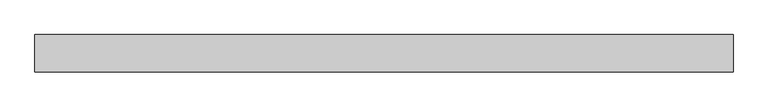
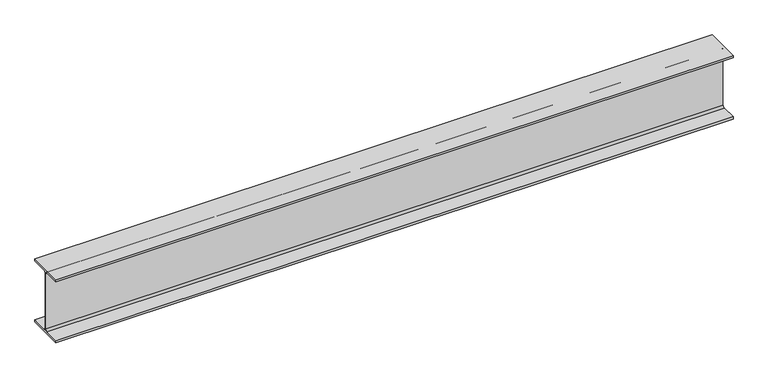
"""IFC4 building model written with IfcOpenShell, lengths in millimetres: beam geometry, Old_Steel Beam_H-KSD3502 : H_SB_ASB_H-300×300x10x15."""

from ifc_helpers import new_model, si_unit, point, frame, frame_2d, origin, place, context, project, spatial, polyline, circle_curve, trimmed, segment, composite_curve, outline, extrude, source, transform, mapped, element, save


def beam_b6f05fa2(model_context):
    return source(origin(), model_context, "Body", "SweptSolid", [
        extrude(outline(composite_curve([segment(polyline([(82.5, -141.5), (82.5, -151.7), (-82.5, -151.7), (-82.5, -141.5), (-11.9, -141.5)]), True, "CONTINUOUS"), segment(trimmed(circle_curve(frame_2d((-11.9, -132.6)), 8.9), [point((-11.9, -141.5))], [point((-3.0, -132.6))], True, "CARTESIAN"), True, "CONTINUOUS"), segment(polyline([(-3.0, -132.6), (-3.0, 132.6)]), True, "CONTINUOUS"), segment(trimmed(circle_curve(frame_2d((-11.9, 132.6)), 8.9), [point((-3.0, 132.6))], [point((-11.9, 141.5))], True, "CARTESIAN"), True, "CONTINUOUS"), segment(polyline([(-11.9, 141.5), (-82.5, 141.5), (-82.5, 151.7), (82.5, 151.7), (82.5, 141.5), (11.9, 141.5)]), True, "CONTINUOUS"), segment(trimmed(circle_curve(frame_2d((11.9, 132.6)), 8.9), [point((11.9, 141.5))], [point((3.0, 132.6))], True, "CARTESIAN"), True, "CONTINUOUS"), segment(polyline([(3.0, 132.6), (3.0, -132.6)]), True, "CONTINUOUS"), segment(trimmed(circle_curve(frame_2d((11.9, -132.6)), 8.9), [point((3.0, -132.6))], [point((11.9, -141.5))], True, "CARTESIAN"), True, "CONTINUOUS"), segment(polyline([(11.9, -141.5), (82.5, -141.5)]), True, "CONTINUOUS")], self_intersect=False)), frame((-1364.2332089, 0.0, 0.0), z_axis=(1.0, 0.0, 0.0), x_axis=(0.0, 1.0, 0.0)), (0.0, 0.0, 1.0), 3068.3751225),
    ])


if __name__ == "__main__":
    model = new_model("IFC4")
    model_context = context("Model", 3, world=origin())
    ifc_project = project(units=[si_unit("LENGTHUNIT", "METRE", prefix="MILLI")], contexts=[model_context])
    site = spatial("IfcSite", under=ifc_project)
    building = spatial("IfcBuilding", under=site)
    placement = place(None, origin())
    beam_shape = beam_b6f05fa2(model_context)
    element("IfcBeam", 1, ObjectType="Old_Steel Beam_H-KSD3502 : H_SB_ASB_H-300×300x10x15", at=placement, inside=building, context=model_context, shape_type="MappedRepresentation", body=[
        mapped(beam_shape, transform((0.0, 0.0, 0.0), x_axis=(1.0, 0.0, 0.0), y_axis=(0.0, 1.0, 0.0), z_axis=(0.0, 0.0, 1.0))),
    ])
    save(model, "model.ifc")

# Revit data of these elements
# Type "Old_Steel Beam_H-KSD3502 : H_SB_ASB_H-300×300x10x15"
#   Width = 30.0 cm
#   Web Thickness = 1.0 cm
#   Web Fillet = 1.8 cm
#   Warping Constant = 1370670.0 cm⁶
#   Torsional Moment of Inertia = 77.00 cm⁴
#   Torsional Modulus = 1.0 cm³
#   Section Area = 119.8 cm²
#   Plastic Modulus weak axis = 684.0 cm³
#   Plastic Modulus strong axis = 1500.0 cm³
#   Perimeter = 1.75 m²/m
#   Nominal Weight = 94.00 kgf/m
#   Moment of Inertia weak axis = 6750.00 cm⁴
#   Moment of Inertia strong axis = 20400.00 cm⁴
#   Height = 30.0 cm
#   Flange Thickness = 1.5 cm
#   Elastic Modulus weak axis = 450.0 cm³
#   Elastic Modulus strong axis = 1360.0 cm³
#   Centroid Vertical = 15.0 cm
#   Centroid Horizontal = 15.0 cm
#   Length [instance default] = 1.5240 m
#   Structural Material [instance default] = Steel, 45-345
#   Assembly Code = ""
# Element 1 (IfcBeam, "Old_Steel Beam_H-KSD3502 : H_SB_ASB_H-300×300x10x15")
#   Structural Material = none
# Materials
#   "Steel, 45-345": class "Metal", colour RGB 189 187 185, transparency 0, Description = "Steel 345 MPa", Cost = 0
